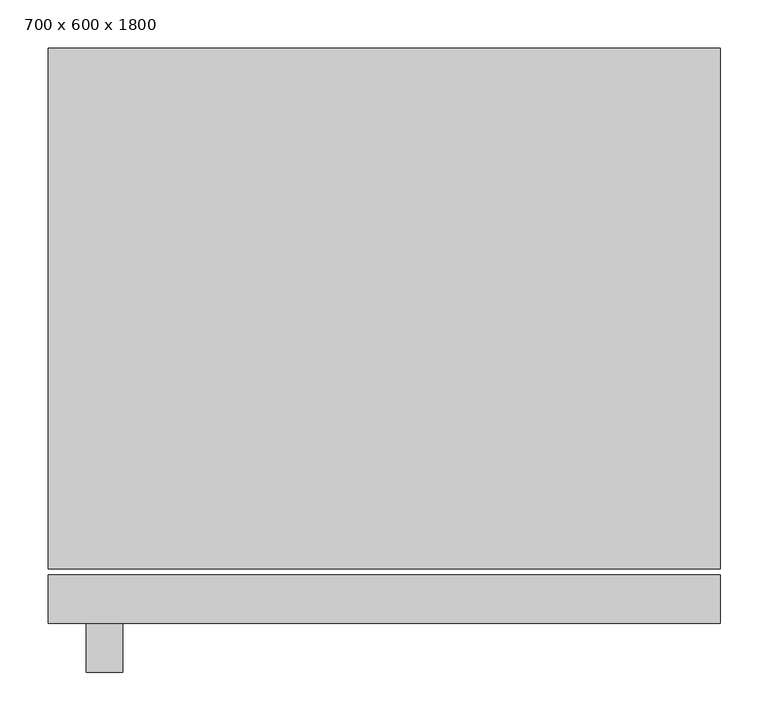
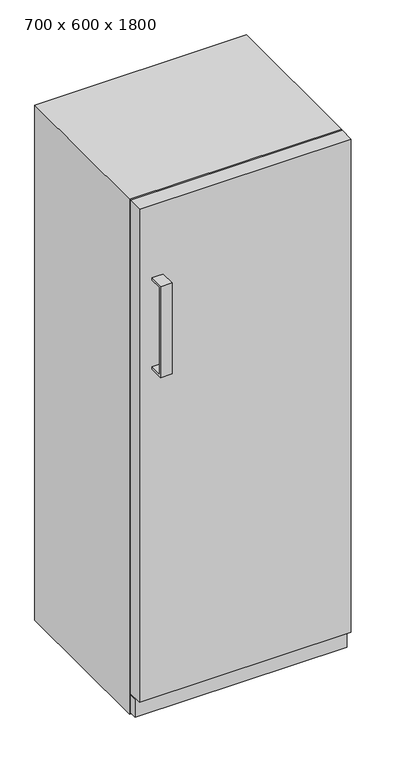
"""IFC4 building model written with IfcOpenShell, lengths in millimetres: furniture geometry, Gefriergerät : 700 x 600 x 1800."""

from ifc_helpers import new_model, si_unit, frame, origin, origin_with_axes, place, context, project, spatial, polyline, outline, extrude, source, transform, mapped, element, save


def furniture_700_x_600_x_1800_e4ec6c65(model_context):
    return source(origin(), model_context, "Body", "SweptSolid", [
        extrude(outline(polyline([(-314.6760285, 1539.65), (-359.1260285, 1539.65), (-359.1260285, 1234.85), (-314.6760285, 1234.85), (-314.6760285, 1228.5154683), (-365.4760285, 1228.5154683), (-365.4760285, 1546.0), (-314.6760285, 1546.0), (-314.6760285, 1539.65)])), frame((-310.0, 0.0, 0.0), z_axis=(1.0, 0.0, 0.0), x_axis=(0.0, 1.0, 0.0)), (0.0, 0.0, 1.0), 38.1),
        extrude(outline(polyline([(350.0, -263.8760285), (350.0, -289.2760285), (-350.0, -289.2760285), (-350.0, -263.8760285), (350.0, -263.8760285)])), frame((0.0, 0.0, 9.3816357), z_axis=(0.0, 0.0, 1.0), x_axis=(1.0, 0.0, 0.0)), (0.0, 0.0, 1.0), 63.5),
        extrude(outline(polyline([(350.0, -263.8760285), (350.0, -314.6760285), (-350.0, -314.6760285), (-350.0, -263.8760285), (350.0, -263.8760285)])), frame((0.0, 0.0, 76.2), z_axis=(0.0, 0.0, 1.0), x_axis=(1.0, 0.0, 0.0)), (0.0, 0.0, 1.0), 1723.8),
        extrude(outline(polyline([(350.0, 285.3239715), (350.0, -257.5260285), (-350.0, -257.5260285), (-350.0, 285.3239715), (350.0, 285.3239715)])), origin_with_axes(), (0.0, 0.0, 1.0), 1800.0),
    ])


if __name__ == "__main__":
    model = new_model("IFC4")
    model_context = context("Model", 3, world=origin())
    ifc_project = project(units=[si_unit("LENGTHUNIT", "METRE", prefix="MILLI")], contexts=[model_context])
    site = spatial("IfcSite", under=ifc_project)
    building = spatial("IfcBuilding", under=site)
    placement = place(None, origin())
    furniture_700_x_600_x_1800_shape = furniture_700_x_600_x_1800_e4ec6c65(model_context)
    element("IfcFurniture", 1, ObjectType="Gefriergerät : 700 x 600 x 1800", at=placement, inside=building, context=model_context, shape_type="MappedRepresentation", body=[
        mapped(furniture_700_x_600_x_1800_shape, transform((0.0, 0.0, 0.0), x_axis=(1.0, 0.0, 0.0), y_axis=(0.0, 1.0, 0.0), z_axis=(0.0, 0.0, 1.0))),
    ])
    save(model, "model.ifc")

# Revit data of these elements
# Type "Gefriergerät : 700 x 600 x 1800"
#   Beschriftung [instance default] = "FRZ"
#   Tiefe = 0.600 m
#   Griff = 0.040 m
#   Höhe = 1.800 m
#   Rückwärtiger Zwischenraum = 0.050 m
#   Breite = 0.700 m
#   Material = Metall - Oberfläche lackiert - Elfenbein - Mit Glanz
#   Assembly Code = ""
# Element 1 (IfcFurniture, "Gefriergerät : 700 x 600 x 1800")
#   Materials on its faces: "Metall - Oberfläche lackiert - Elfenbein - Mit Glanz", "Metall - Chrom", "Metall - Oberfläche bemalt - Schwarz mit Glanz"
# Materials
#   "Metall - Oberfläche lackiert - Elfenbein - Mit Glanz": class "Farbe 1", colour RGB 247 247 239, transparency 0
#   "Metall - Chrom": class "Metall", colour RGB 247 247 247, transparency 0, Cost = 0
#   "Metall - Oberfläche bemalt - Schwarz mit Glanz": class "Farbe 1", colour RGB 0 0 0, transparency 0
